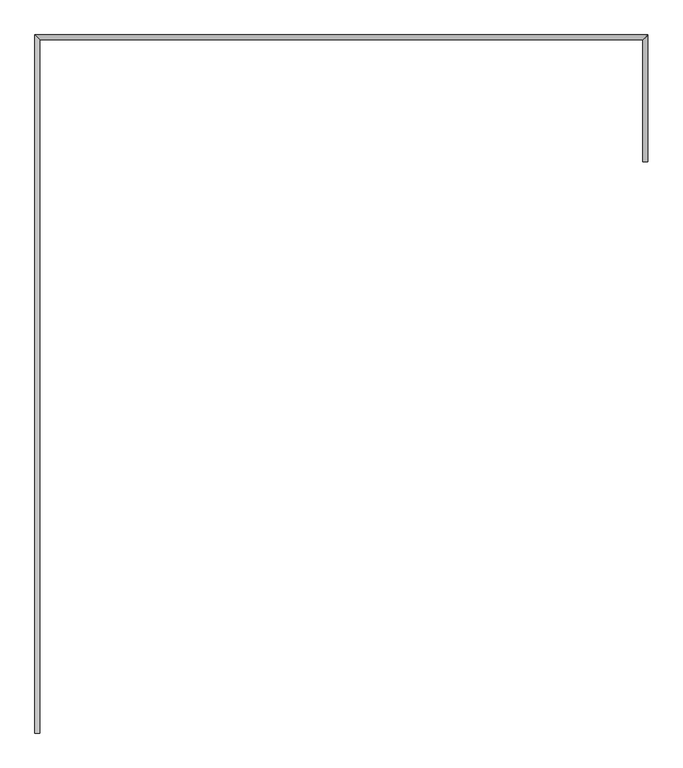
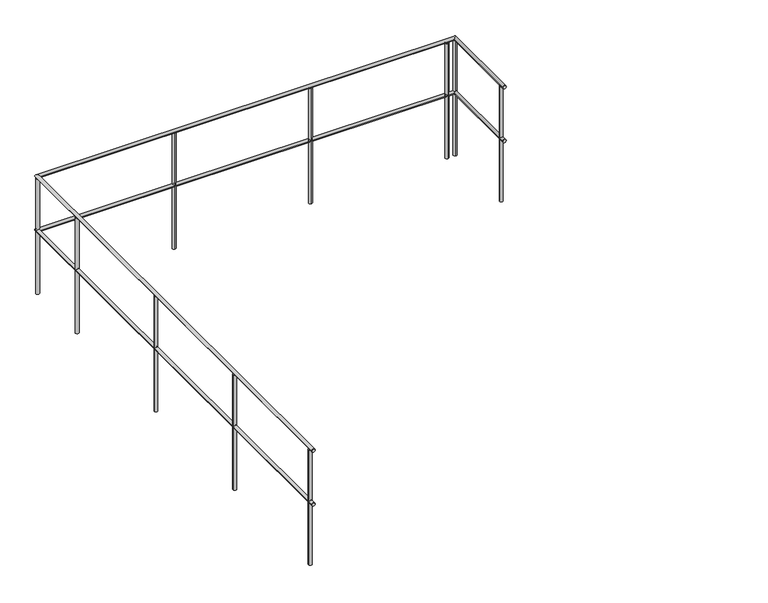
"""IFC4 building model written with IfcOpenShell, lengths in millimetres: railing geometry."""

from ifc_helpers import new_model, si_unit, point, frame, frame_2d, origin, place, context, project, spatial, circle_curve, ellipse_curve, trimmed, segment, composite_curve, outline, extrude, source, transform, mapped, element, save
from ifc_brep_helpers import plane_surface, cylinder_surface, advanced_brep


def railing_4f0946f5(model_context):
    return source(origin(), model_context, "Body", "SolidModel", [
        advanced_brep(
        [(-4051.0, 57498.9598198, 885.0), (-4081.0, 57498.9598198, 885.0), (-4081.0, 61717.0208589, 885.0), (-4051.0, 61687.0208589, 885.0), (-377.8127408, 61717.0208589, 885.0), (-407.8127408, 61687.0208589, 885.0), (-407.8127408, 60949.5208589, 885.0), (-377.8127408, 60949.5208589, 885.0)],
        [
            (0, 1, circle_curve(frame((-4066.0, 57498.9598198, 885.0), z_axis=(0.0, -1.0, 0.0), x_axis=(-1.0, 0.0, 0.0)), 15.0)),
            (1, 0, circle_curve(frame((-4066.0, 57498.9598198, 885.0), z_axis=(0.0, -1.0, 0.0), x_axis=(-1.0, 0.0, 0.0)), 15.0)),
            (1, 2),
            (2, 3, ellipse_curve(frame((-4066.0, 61702.0208589, 885.0), z_axis=(-0.7071067811865489, -0.707106781186546, 0.0), x_axis=(0.707106781186546, -0.7071067811865491, 0.0)), 21.2132034, 15.0)),
            (3, 0),
            (3, 2, ellipse_curve(frame((-4066.0, 61702.0208589, 885.0), z_axis=(-0.7071067811865489, -0.707106781186546, 0.0), x_axis=(0.707106781186546, -0.7071067811865491, 0.0)), 21.2132034, 15.0)),
            (2, 4),
            (4, 5, ellipse_curve(frame((-392.8127408, 61702.0208589, 885.0), z_axis=(-0.707106781186546, 0.707106781186549, 0.0), x_axis=(-0.707106781186549, -0.707106781186546, 0.0)), 21.2132034, 15.0)),
            (5, 3),
            (5, 4, ellipse_curve(frame((-392.8127408, 61702.0208589, 885.0), z_axis=(-0.707106781186546, 0.707106781186549, 0.0), x_axis=(-0.707106781186549, -0.707106781186546, 0.0)), 21.2132034, 15.0)),
            (6, 7, circle_curve(frame((-392.8127408, 60949.5208589, 885.0), z_axis=(0.0, -1.0, 0.0), x_axis=(1.0, 0.0, 0.0)), 15.0)),
            (7, 6, circle_curve(frame((-392.8127408, 60949.5208589, 885.0), z_axis=(0.0, -1.0, 0.0), x_axis=(1.0, 0.0, 0.0)), 15.0)),
            (4, 7),
            (6, 5),
        ],
        [
            plane_surface(frame((-4066.0, 57498.9598198, 900.0), z_axis=(0.0, -1.0, 0.0), x_axis=(0.0, 0.0, 1.0))),
            cylinder_surface(frame((-4066.0, 57498.9598198, 885.0), z_axis=(0.0, -1.0, 0.0), x_axis=(-1.0, 0.0, 0.0)), 15.0),
            cylinder_surface(frame((-4066.0, 61702.0208589, 885.0), z_axis=(-1.0, 0.0, 0.0), x_axis=(0.0, 1.0, 0.0)), 15.0),
            plane_surface(frame((-392.8127408, 60949.5208589, 900.0), z_axis=(0.0, -1.0, 0.0), x_axis=(0.0, 0.0, -1.0))),
            cylinder_surface(frame((-392.8127408, 61702.0208589, 885.0), z_axis=(0.0, 1.0, 0.0), x_axis=(1.0, 0.0, 0.0)), 15.0),
        ],
        [
            (0, [[1, 2]]),
            (1, [[-2, 3, 4, 5]]),
            (1, [[-1, -5, 6, -3]]),
            (2, [[-4, 7, 8, 9]]),
            (2, [[-6, -9, 10, -7]]),
            (3, [[11, 12]]),
            (4, [[-8, 13, -11, 14]]),
            (4, [[-10, -14, -12, -13]]),
        ],
    ),
        advanced_brep(
        [(-4051.0, 57498.9598198, 1385.0), (-4081.0, 57498.9598198, 1385.0), (-4081.0, 61717.0208589, 1385.0), (-4051.0, 61687.0208589, 1385.0), (-377.8127408, 61717.0208589, 1385.0), (-407.8127408, 61687.0208589, 1385.0), (-407.8127408, 60949.5208589, 1385.0), (-377.8127408, 60949.5208589, 1385.0)],
        [
            (0, 1, circle_curve(frame((-4066.0, 57498.9598198, 1385.0), z_axis=(0.0, -1.0, 0.0), x_axis=(-1.0, 0.0, 0.0)), 15.0)),
            (1, 0, circle_curve(frame((-4066.0, 57498.9598198, 1385.0), z_axis=(0.0, -1.0, 0.0), x_axis=(-1.0, 0.0, 0.0)), 15.0)),
            (1, 2),
            (2, 3, ellipse_curve(frame((-4066.0, 61702.0208589, 1385.0), z_axis=(-0.7071067811865489, -0.707106781186546, 0.0), x_axis=(0.707106781186546, -0.7071067811865491, 0.0)), 21.2132034, 15.0)),
            (3, 0),
            (3, 2, ellipse_curve(frame((-4066.0, 61702.0208589, 1385.0), z_axis=(-0.7071067811865489, -0.707106781186546, 0.0), x_axis=(0.707106781186546, -0.7071067811865491, 0.0)), 21.2132034, 15.0)),
            (2, 4),
            (4, 5, ellipse_curve(frame((-392.8127408, 61702.0208589, 1385.0), z_axis=(-0.707106781186546, 0.707106781186549, 0.0), x_axis=(-0.707106781186549, -0.707106781186546, 0.0)), 21.2132034, 15.0)),
            (5, 3),
            (5, 4, ellipse_curve(frame((-392.8127408, 61702.0208589, 1385.0), z_axis=(-0.707106781186546, 0.707106781186549, 0.0), x_axis=(-0.707106781186549, -0.707106781186546, 0.0)), 21.2132034, 15.0)),
            (6, 7, circle_curve(frame((-392.8127408, 60949.5208589, 1385.0), z_axis=(0.0, -1.0, 0.0), x_axis=(1.0, 0.0, 0.0)), 15.0)),
            (7, 6, circle_curve(frame((-392.8127408, 60949.5208589, 1385.0), z_axis=(0.0, -1.0, 0.0), x_axis=(1.0, 0.0, 0.0)), 15.0)),
            (4, 7),
            (6, 5),
        ],
        [
            plane_surface(frame((-4066.0, 57498.9598198, 1400.0), z_axis=(0.0, -1.0, 0.0), x_axis=(0.0, 0.0, 1.0))),
            cylinder_surface(frame((-4066.0, 57498.9598198, 1385.0), z_axis=(0.0, -1.0, 0.0), x_axis=(-1.0, 0.0, 0.0)), 15.0),
            cylinder_surface(frame((-4066.0, 61702.0208589, 1385.0), z_axis=(-1.0, 0.0, 0.0), x_axis=(0.0, 1.0, 0.0)), 15.0),
            plane_surface(frame((-392.8127408, 60949.5208589, 1400.0), z_axis=(0.0, -1.0, 0.0), x_axis=(0.0, 0.0, -1.0))),
            cylinder_surface(frame((-392.8127408, 61702.0208589, 1385.0), z_axis=(0.0, 1.0, 0.0), x_axis=(1.0, 0.0, 0.0)), 15.0),
        ],
        [
            (0, [[1, 2]]),
            (1, [[-2, 3, 4, 5]]),
            (1, [[-1, -5, 6, -3]]),
            (2, [[-4, 7, 8, 9]]),
            (2, [[-6, -9, 10, -7]]),
            (3, [[11, 12]]),
            (4, [[-8, 13, -11, 14]]),
            (4, [[-10, -14, -12, -13]]),
        ],
    ),
        extrude(outline(composite_curve([segment(trimmed(circle_curve(frame_2d((-466.0, 61702.0208589)), 15.0), [point((-466.0, 61687.0208589))], [point((-466.0, 61717.0208589))], False, "CARTESIAN"), True, "CONTINUOUS"), segment(trimmed(circle_curve(frame_2d((-466.0, 61702.0208589)), 15.0), [point((-466.0, 61717.0208589))], [point((-466.0, 61687.0208589))], False, "CARTESIAN"), True, "CONTINUOUS")], self_intersect=False)), frame((0.0, 0.0, 300.0), z_axis=(0.0, 0.0, 1.0), x_axis=(1.0, 0.0, 0.0)), (0.0, 0.0, 1.0), 1070.0),
        extrude(outline(composite_curve([segment(trimmed(circle_curve(frame_2d((-1666.0, 61702.0208589)), 15.0), [point((-1666.0, 61687.0208589))], [point((-1666.0, 61717.0208589))], False, "CARTESIAN"), True, "CONTINUOUS"), segment(trimmed(circle_curve(frame_2d((-1666.0, 61702.0208589)), 15.0), [point((-1666.0, 61717.0208589))], [point((-1666.0, 61687.0208589))], False, "CARTESIAN"), True, "CONTINUOUS")], self_intersect=False)), frame((0.0, 0.0, 300.0), z_axis=(0.0, 0.0, 1.0), x_axis=(1.0, 0.0, 0.0)), (0.0, 0.0, 1.0), 1070.0),
        extrude(outline(composite_curve([segment(trimmed(circle_curve(frame_2d((-2866.0, 61702.0208589)), 15.0), [point((-2866.0, 61687.0208589))], [point((-2866.0, 61717.0208589))], False, "CARTESIAN"), True, "CONTINUOUS"), segment(trimmed(circle_curve(frame_2d((-2866.0, 61702.0208589)), 15.0), [point((-2866.0, 61717.0208589))], [point((-2866.0, 61687.0208589))], False, "CARTESIAN"), True, "CONTINUOUS")], self_intersect=False)), frame((0.0, 0.0, 300.0), z_axis=(0.0, 0.0, 1.0), x_axis=(1.0, 0.0, 0.0)), (0.0, 0.0, 1.0), 1070.0),
        extrude(outline(composite_curve([segment(trimmed(circle_curve(frame_2d((-4066.0, 61098.9598198)), 15.0), [point((-4051.0, 61098.9598198))], [point((-4081.0, 61098.9598198))], False, "CARTESIAN"), True, "CONTINUOUS"), segment(trimmed(circle_curve(frame_2d((-4066.0, 61098.9598198)), 15.0), [point((-4081.0, 61098.9598198))], [point((-4051.0, 61098.9598198))], False, "CARTESIAN"), True, "CONTINUOUS")], self_intersect=False)), frame((0.0, 0.0, 300.0), z_axis=(0.0, 0.0, 1.0), x_axis=(1.0, 0.0, 0.0)), (0.0, 0.0, 1.0), 1070.0),
        extrude(outline(composite_curve([segment(trimmed(circle_curve(frame_2d((-4066.0, 59898.9598198)), 15.0), [point((-4051.0, 59898.9598198))], [point((-4081.0, 59898.9598198))], False, "CARTESIAN"), True, "CONTINUOUS"), segment(trimmed(circle_curve(frame_2d((-4066.0, 59898.9598198)), 15.0), [point((-4081.0, 59898.9598198))], [point((-4051.0, 59898.9598198))], False, "CARTESIAN"), True, "CONTINUOUS")], self_intersect=False)), frame((0.0, 0.0, 300.0), z_axis=(0.0, 0.0, 1.0), x_axis=(1.0, 0.0, 0.0)), (0.0, 0.0, 1.0), 1070.0),
        extrude(outline(composite_curve([segment(trimmed(circle_curve(frame_2d((-4066.0, 58698.9598198)), 15.0), [point((-4051.0, 58698.9598198))], [point((-4081.0, 58698.9598198))], False, "CARTESIAN"), True, "CONTINUOUS"), segment(trimmed(circle_curve(frame_2d((-4066.0, 58698.9598198)), 15.0), [point((-4081.0, 58698.9598198))], [point((-4051.0, 58698.9598198))], False, "CARTESIAN"), True, "CONTINUOUS")], self_intersect=False)), frame((0.0, 0.0, 300.0), z_axis=(0.0, 0.0, 1.0), x_axis=(1.0, 0.0, 0.0)), (0.0, 0.0, 1.0), 1070.0),
        extrude(outline(composite_curve([segment(trimmed(circle_curve(frame_2d((-392.8127408, 61702.0208589)), 15.0), [point((-392.8127408, 61687.0208589))], [point((-392.8127408, 61717.0208589))], False, "CARTESIAN"), True, "CONTINUOUS"), segment(trimmed(circle_curve(frame_2d((-392.8127408, 61702.0208589)), 15.0), [point((-392.8127408, 61717.0208589))], [point((-392.8127408, 61687.0208589))], False, "CARTESIAN"), True, "CONTINUOUS")], self_intersect=False)), frame((0.0, 0.0, 300.0), z_axis=(0.0, 0.0, 1.0), x_axis=(1.0, 0.0, 0.0)), (0.0, 0.0, 1.0), 1070.0),
        extrude(outline(composite_curve([segment(trimmed(circle_curve(frame_2d((-4066.0, 61702.0208589)), 15.0), [point((-4051.0, 61702.0208589))], [point((-4081.0, 61702.0208589))], False, "CARTESIAN"), True, "CONTINUOUS"), segment(trimmed(circle_curve(frame_2d((-4066.0, 61702.0208589)), 15.0), [point((-4081.0, 61702.0208589))], [point((-4051.0, 61702.0208589))], False, "CARTESIAN"), True, "CONTINUOUS")], self_intersect=False)), frame((0.0, 0.0, 300.0), z_axis=(0.0, 0.0, 1.0), x_axis=(1.0, 0.0, 0.0)), (0.0, 0.0, 1.0), 1070.0),
        extrude(outline(composite_curve([segment(trimmed(circle_curve(frame_2d((-392.8127408, 60999.5208589)), 15.0), [point((-407.8127408, 60999.5208589))], [point((-377.8127408, 60999.5208589))], False, "CARTESIAN"), True, "CONTINUOUS"), segment(trimmed(circle_curve(frame_2d((-392.8127408, 60999.5208589)), 15.0), [point((-377.8127408, 60999.5208589))], [point((-407.8127408, 60999.5208589))], False, "CARTESIAN"), True, "CONTINUOUS")], self_intersect=False)), frame((0.0, 0.0, 300.0), z_axis=(0.0, 0.0, 1.0), x_axis=(1.0, 0.0, 0.0)), (0.0, 0.0, 1.0), 1070.0),
        extrude(outline(composite_curve([segment(trimmed(circle_curve(frame_2d((-4066.0, 57548.9598198)), 15.0), [point((-4051.0, 57548.9598198))], [point((-4081.0, 57548.9598198))], False, "CARTESIAN"), True, "CONTINUOUS"), segment(trimmed(circle_curve(frame_2d((-4066.0, 57548.9598198)), 15.0), [point((-4081.0, 57548.9598198))], [point((-4051.0, 57548.9598198))], False, "CARTESIAN"), True, "CONTINUOUS")], self_intersect=False)), frame((0.0, 0.0, 300.0), z_axis=(0.0, 0.0, 1.0), x_axis=(1.0, 0.0, 0.0)), (0.0, 0.0, 1.0), 1070.0),
    ])


if __name__ == "__main__":
    model = new_model("IFC4")
    model_context = context("Model", 3, world=origin())
    ifc_project = project(units=[si_unit("LENGTHUNIT", "METRE", prefix="MILLI")], contexts=[model_context])
    site = spatial("IfcSite", under=ifc_project)
    building = spatial("IfcBuilding", under=site)
    placement = place(None, origin())
    railing_shape = railing_4f0946f5(model_context)
    element("IfcRailing", 1, at=placement, inside=building, context=model_context, shape_type="MappedRepresentation", body=[
        mapped(railing_shape, transform((0.0, 0.0, 0.0), x_axis=(1.0, 0.0, 0.0), y_axis=(0.0, 1.0, 0.0), z_axis=(0.0, 0.0, 1.0))),
    ])
    save(model, "model.ifc")
